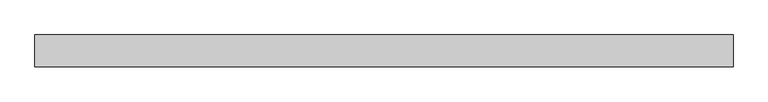
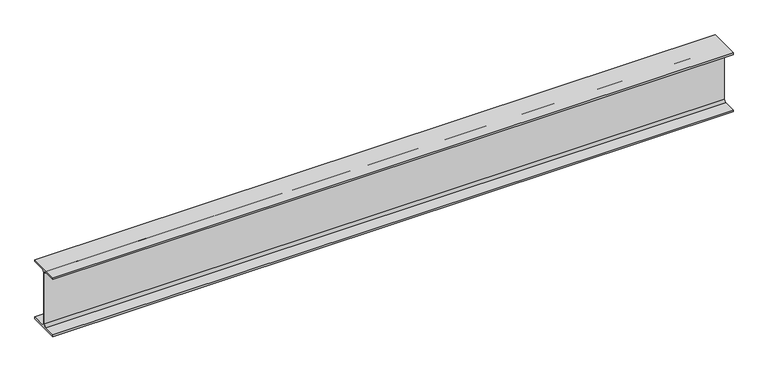
"""IFC4 building model written with IfcOpenShell, lengths in millimetres: beam geometry, 0912_Steel Framing_H-KSD3502 : H_SB_ASB_H-350x175x7x11."""

from ifc_helpers import new_model, si_unit, point, frame, frame_2d, origin, place, context, project, spatial, polyline, circle_curve, trimmed, segment, composite_curve, outline, extrude, source, transform, mapped, element, save


def beam_2fbc9c0e(model_context):
    return source(origin(), model_context, "Body", "SweptSolid", [
        extrude(outline(composite_curve([segment(polyline([(87.5, -164.0), (87.5, -175.0), (-87.5, -175.0), (-87.5, -164.0), (-17.5, -164.0)]), True, "CONTINUOUS"), segment(trimmed(circle_curve(frame_2d((-17.5, -150.0)), 14.0), [point((-17.5, -164.0))], [point((-3.5, -150.0))], True, "CARTESIAN"), True, "CONTINUOUS"), segment(polyline([(-3.5, -150.0), (-3.5, 150.0)]), True, "CONTINUOUS"), segment(trimmed(circle_curve(frame_2d((-17.5, 150.0)), 14.0), [point((-3.5, 150.0))], [point((-17.5, 164.0))], True, "CARTESIAN"), True, "CONTINUOUS"), segment(polyline([(-17.5, 164.0), (-87.5, 164.0), (-87.5, 175.0), (87.5, 175.0), (87.5, 164.0), (17.5, 164.0)]), True, "CONTINUOUS"), segment(trimmed(circle_curve(frame_2d((17.5, 150.0)), 14.0), [point((17.5, 164.0))], [point((3.5, 150.0))], True, "CARTESIAN"), True, "CONTINUOUS"), segment(polyline([(3.5, 150.0), (3.5, -150.0)]), True, "CONTINUOUS"), segment(trimmed(circle_curve(frame_2d((17.5, -150.0)), 14.0), [point((3.5, -150.0))], [point((17.5, -164.0))], True, "CARTESIAN"), True, "CONTINUOUS"), segment(polyline([(17.5, -164.0), (87.5, -164.0)]), True, "CONTINUOUS")], self_intersect=False)), frame((-1904.8, 0.0, 0.0), z_axis=(1.0, 0.0, 0.0), x_axis=(0.0, 1.0, 0.0)), (0.0, 0.0, 1.0), 3809.6),
    ])


if __name__ == "__main__":
    model = new_model("IFC4")
    model_context = context("Model", 3, world=origin())
    ifc_project = project(units=[si_unit("LENGTHUNIT", "METRE", prefix="MILLI")], contexts=[model_context])
    site = spatial("IfcSite", under=ifc_project)
    building = spatial("IfcBuilding", under=site)
    placement = place(None, origin())
    beam_shape = beam_2fbc9c0e(model_context)
    element("IfcBeam", 1, ObjectType="0912_Steel Framing_H-KSD3502 : H_SB_ASB_H-350x175x7x11", at=placement, inside=building, context=model_context, shape_type="MappedRepresentation", body=[
        mapped(beam_shape, transform((0.0, 0.0, 0.0), x_axis=(1.0, 0.0, 0.0), y_axis=(0.0, 1.0, 0.0), z_axis=(0.0, 0.0, 1.0))),
    ])
    save(model, "model.ifc")

# Revit data of these elements
# Type "0912_Steel Framing_H-KSD3502 : H_SB_ASB_H-350x175x7x11"
#   H_WM Code_1 = "S01AA002-00001 | Main Steel Structure Fabrication Work | Shelter/Building | Medium Steel - Standard (90KG/M>Weight≥30KG/M) | Material: (   )"
#   H_WM Code_2 = "S03AA028-00001 | Main Steel Structure Erection Work | Shelter/Building | Medium Steel (90KG/M>Weight≥30KG/M) | Material: (   )"
#   H_WM Code_3 = "S01AA010-00001 | Main Steel Structure Fabrication Work | Shelter/Building | Steel Painting/Coating | for Non-Fireproofed Steel Surface, Surface Preparation, Primer, Second & Final Coat | Material: (   )"
#   H_Q'ty Cal Type Tag = "SB-Q2"
#   Width = 17.5 cm
#   Web Thickness = 0.7 cm
#   Web Fillet = 1.4 cm
#   Warping Constant = 282000.0 cm⁶
#   W = 0
#   Torsional Moment of Inertia = 19.4042 cm⁴
#   Section Area = 63.14 cm²
#   Plastic Modulus weak axis = 174.0 cm³
#   Plastic Modulus strong axis = 868.0 cm³
#   Perimeter = 1.36 m²/m
#   Nominal Weight = 49.60 kgf/m
#   Moment of Inertia weak axis = 984.00 cm⁴
#   Moment of Inertia strong axis = 13600.00 cm⁴
#   Height = 35.0 cm
#   Flange Thickness = 1.1 cm
#   Elastic Modulus weak axis = 112.0 cm³
#   Elastic Modulus strong axis = 775.0 cm³
#   Centroid Vertical = 17.5 cm
#   Centroid Horizontal = 8.75 cm
#   Ix = 136000000
#   Length [instance default] = 1.5240 m
#   Zx = 868000
#   b = 0.1750 m
#   h = 0.3500 m
#   r = 0.0140 m
#   s = 0.0070 m
#   t = 0.0110 m
#   A = 0.006314 m²
#   Structural Material [instance default] = Steel, 45-345
#   Assembly Code = ""
# Element 1 (IfcBeam, "0912_Steel Framing_H-KSD3502 : H_SB_ASB_H-350x175x7x11")
#   Structural Material = none
# Materials
#   "Steel, 45-345": class "Metal", colour RGB 189 187 185, transparency 0, Description = "Steel 345 MPa", Cost = 0
